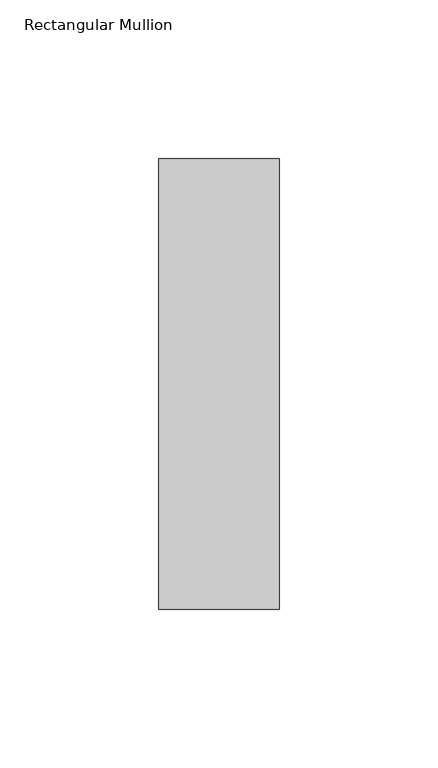
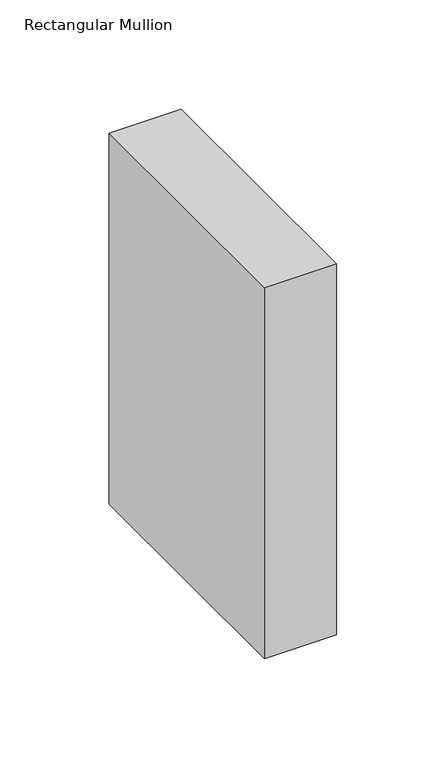
"""IFC4 building model written with IfcOpenShell, lengths in millimetres: member geometry, Rectangular Mullion : NLRS_21_CWM_hsb-regel 38x142_gen_rsf."""

from ifc_helpers import new_model, si_unit, frame, origin, place, context, project, spatial, polyline, outline, extrude, source, transform, mapped, element, save


def rectangular_mullion_ed461cf7(model_context):
    return source(origin(), model_context, "Body", "SweptSolid", [
        extrude(outline(polyline([(0.0, -71.0), (-38.0, -71.0), (-38.0, 71.0), (0.0, 71.0), (0.0, -71.0)])), frame((0.0, 0.0, -207.0000003), z_axis=(0.0, 0.0, 1.0), x_axis=(1.0, 0.0, 0.0)), (0.0, 0.0, 1.0), 207.0000003),
    ])


if __name__ == "__main__":
    model = new_model("IFC4")
    model_context = context("Model", 3, world=origin())
    ifc_project = project(units=[si_unit("LENGTHUNIT", "METRE", prefix="MILLI")], contexts=[model_context])
    site = spatial("IfcSite", under=ifc_project)
    building = spatial("IfcBuilding", under=site)
    placement = place(None, origin())
    rectangular_mullion_shape = rectangular_mullion_ed461cf7(model_context)
    element("IfcMember", 1, ObjectType="Rectangular Mullion : NLRS_21_CWM_hsb-regel 38x142_gen_rsf", at=placement, inside=building, context=model_context, shape_type="MappedRepresentation", body=[
        mapped(rectangular_mullion_shape, transform((0.0, 0.0, 0.0), x_axis=(1.0, 0.0, 0.0), y_axis=(0.0, 1.0, 0.0), z_axis=(0.0, 0.0, 1.0))),
    ])
    save(model, "model.ifc")

# Revit data of these elements
# Type "Rectangular Mullion : NLRS_21_CWM_hsb-regel 38x142_gen_rsf"
#   Export Type to IFC As = "IfcWall"
#   Type IfcGUID = "07M7mRoiH1CR8m_RSKIwpF"
#   Assembly Code = "21.10"
#   built-in parameter 1007322 = 0.465879 (stored number, unit not read)
#   built-in parameter 1007321 = 0.062336 (stored number, unit not read)
#   built-in parameter 1007320 = 0.062336 (stored number, unit not read)
# Element 1 (IfcMember, "Rectangular Mullion : NLRS_21_CWM_hsb-regel 38x142_gen_rsf")
#   Materials on its faces: "NLRS_i2_hout naaldhout vuren_gen_rsf"
# Materials
#   "NLRS_i2_hout naaldhout vuren_gen_rsf": class "I - Hout", colour RGB 234 199 147, transparency 0, Keynote = "i2", Manufacturer = "Revit Standards Foundation", URL = "www.revitstandards.org", Description = "hout vuren", Cost = 0
